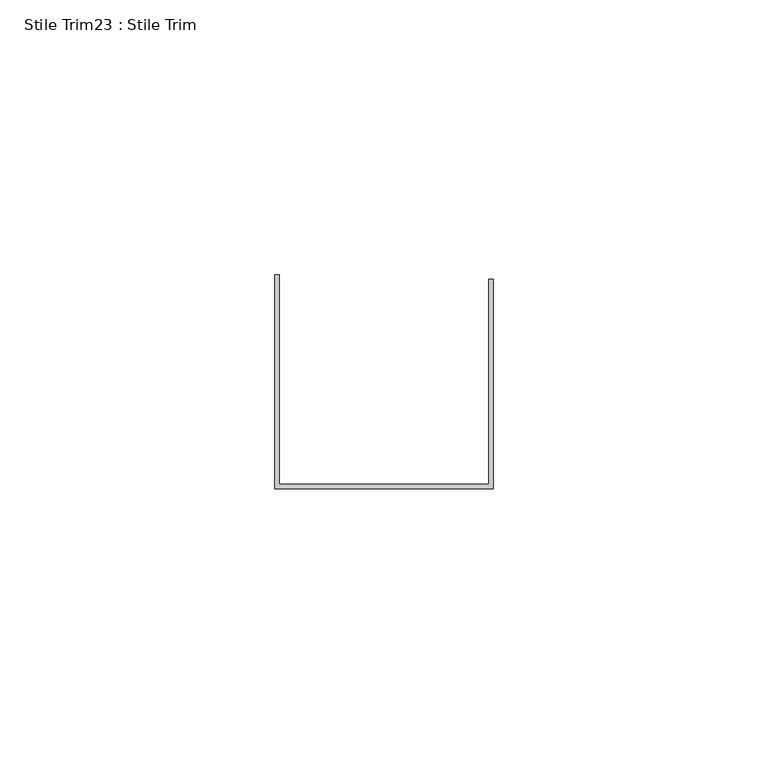
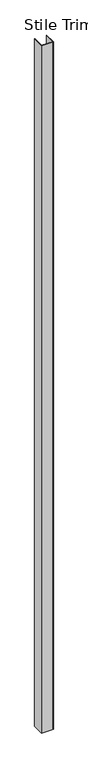
"""IFC4 building model written with IfcOpenShell, lengths in millimetres: proxy geometry, Stile Trim23 : Stile Trim."""

from ifc_helpers import new_model, si_unit, frame, origin, place, context, project, spatial, polyline, outline, extrude, source, transform, mapped, element, save


def stile_trim23_stile_trim_c821ec75(model_context):
    return source(origin(), model_context, "Body", "SweptSolid", [
        extrude(outline(polyline([(587327.0060739, -534097.4537841), (587327.0060739, -534058.5663841), (587327.7934739, -534058.5663841), (587327.7934739, -534096.6663841), (587365.8934739, -534096.6663841), (587365.8934739, -534059.3537841), (587366.6808739, -534059.3537841), (587366.6808739, -534097.4537841), (587327.0060739, -534097.4537841)])), frame((0.0, 0.0, 12.7), z_axis=(0.0, 0.0, 1.0), x_axis=(1.0, 0.0, 0.0)), (0.0, 0.0, 1.0), 2425.7),
    ])


if __name__ == "__main__":
    model = new_model("IFC4")
    model_context = context("Model", 3, world=origin())
    ifc_project = project(units=[si_unit("LENGTHUNIT", "METRE", prefix="MILLI")], contexts=[model_context])
    site = spatial("IfcSite", under=ifc_project)
    building = spatial("IfcBuilding", under=site)
    placement = place(None, origin())
    stile_trim23_stile_trim_shape = stile_trim23_stile_trim_c821ec75(model_context)
    element("IfcBuildingElementProxy", 1, Name="Stile Trim23 : Stile Trim", ObjectType="Stile Trim23 : Stile Trim", at=placement, inside=building, context=model_context, shape_type="MappedRepresentation", body=[
        mapped(stile_trim23_stile_trim_shape, transform((0.0, 0.0, 0.0), x_axis=(1.0, 0.0, 0.0), y_axis=(0.0, 1.0, 0.0), z_axis=(0.0, 0.0, 1.0))),
    ])
    save(model, "model.ifc")

# Revit data of these elements
# Element 1 (IfcBuildingElementProxy, "Stile Trim23 : Stile Trim")
#   Materials on its faces: "EDGE TRIM BY MTL PANEL MFR."
# Materials
#   "EDGE TRIM BY MTL PANEL MFR.": class "Generic", colour RGB 239 242 240, transparency 0, Cost = 0
